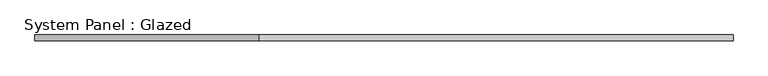
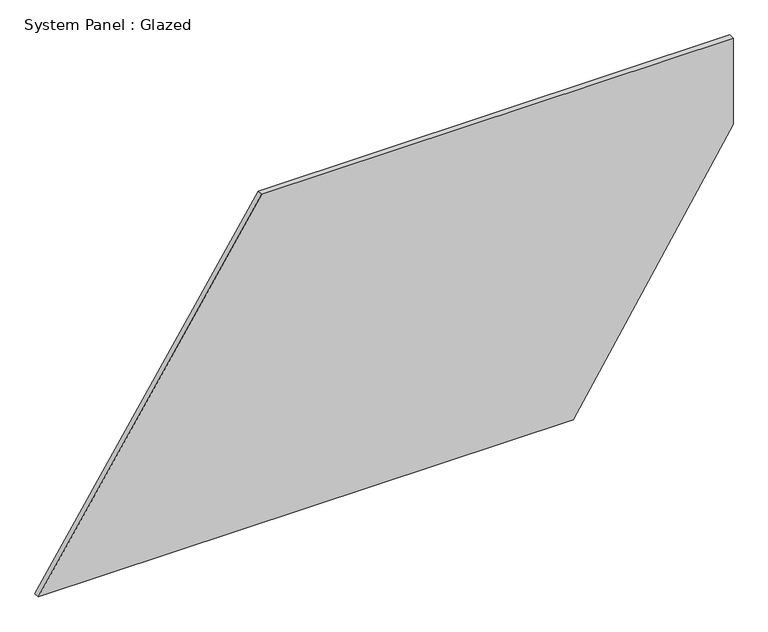
"""IFC4 building model written with IfcOpenShell, lengths in millimetres: plate geometry, System Panel : Glazed."""

import ifcopenshell
import ifcopenshell.guid

model = None  # the IFC model being written
_history = None  # IfcOwnerHistory: only IFC2X3 demands one
_inside = {}  # id of a spatial element -> (the spatial element, [elements in it])
_under = {}  # id of a project, library or spatial element -> (it, [spatial elements below it])
_declared = {}  # id of a project -> (the project, [libraries it declares])
_typed = {}  # id of a type object -> (the type object, [elements of that type])
_made_of = {}  # id of a material, layer set ... -> (it, [elements and type objects made of it])


def new_model(schema):
    """Start an empty IFC model of exactly this schema.

    Asked for "IFC4X3", IfcOpenShell would pick the latest addendum, in which some entities
    have other attributes; the version numbers below select the first issue.
    IFC2X3 requires an IfcOwnerHistory on every rooted entity: one is made here for all.
    """
    global model, _history
    if schema == "IFC4X3":
        model = ifcopenshell.file(schema_version=(4, 3, 0, 0))
    else:
        model = ifcopenshell.file(schema=schema)
    _inside.clear()
    _under.clear()
    _declared.clear()
    _typed.clear()
    _made_of.clear()
    _history = None
    if model.schema == "IFC2X3":
        org = make("IfcOrganization", Name="unknown")
        user = make(
            "IfcPersonAndOrganization",
            ThePerson=make("IfcPerson", FamilyName="unknown"),
            TheOrganization=org,
        )
        app = make(
            "IfcApplication",
            ApplicationDeveloper=org,
            Version="unknown",
            ApplicationFullName="unknown",
            ApplicationIdentifier="unknown",
        )
        _history = make(
            "IfcOwnerHistory",
            OwningUser=user,
            OwningApplication=app,
            ChangeAction="ADDED",
            CreationDate=0,
        )
    return model


def make(cls, **values):
    """One entity of the class cls with the attributes given. An attribute that is None is left unset."""
    return model.create_entity(
        cls, **{name: value for name, value in values.items() if value is not None}
    )


def rooted(cls, **values):
    """An entity with a GlobalId (a new one), such as an element, a storey or a relation."""
    return make(cls, GlobalId=ifcopenshell.guid.new(), OwnerHistory=_history, **values)


def si_unit(unit_type, name, prefix=None):
    """IfcSIUnit, for example si_unit("LENGTHUNIT", "METRE", prefix="MILLI")."""
    return make("IfcSIUnit", UnitType=unit_type, Prefix=prefix, Name=name)


def assignment(units):
    """IfcUnitAssignment: the units of a project."""
    return None if units is None else make("IfcUnitAssignment", Units=units)


def point(xyz):
    """IfcCartesianPoint."""
    return None if xyz is None else make("IfcCartesianPoint", Coordinates=xyz)


def direction(xyz):
    """IfcDirection."""
    return None if xyz is None else make("IfcDirection", DirectionRatios=xyz)


def frame(location, z_axis=None, x_axis=None):
    """IfcAxis2Placement3D, a coordinate frame: its origin and axes. An axis left out is left unset."""
    return make(
        "IfcAxis2Placement3D",
        Location=point(location),
        Axis=direction(z_axis),
        RefDirection=direction(x_axis),
    )


def origin():
    """The frame at (0, 0, 0) with its axes left unset."""
    return frame((0.0, 0.0, 0.0))


def place(relative_to, where):
    """IfcLocalPlacement: puts the frame where relative to a parent placement (None: the world)."""
    return make(
        "IfcLocalPlacement", PlacementRelTo=relative_to, RelativePlacement=where
    )


def context(
    kind, dimensions, precision=None, world=None, true_north=None, identifier=None
):
    """IfcGeometricRepresentationContext, for example the 3D "Model" context."""
    return make(
        "IfcGeometricRepresentationContext",
        ContextIdentifier=identifier,
        ContextType=kind,
        CoordinateSpaceDimension=dimensions,
        Precision=precision,
        WorldCoordinateSystem=world,
        TrueNorth=true_north,
    )


def project(units=None, contexts=None):
    """IfcProject with its units and contexts."""
    return rooted(
        "IfcProject",
        Name="project",
        RepresentationContexts=contexts,
        UnitsInContext=assignment(units),
    )


def spatial(cls, under=None, at=None, **own):
    """A site, building, storey or space (cls), placed at a placement, below another one or the project."""
    s = rooted(cls, ObjectPlacement=at, **own)
    if under is not None:
        _under.setdefault(under.id(), (under, []))[1].append(s)
    return s


def polyline(points):
    """IfcPolyline through the points."""
    return make("IfcPolyline", Points=[point(p) for p in points])


def outline(outer, holes=None, kind="AREA"):
    """IfcArbitraryClosedProfileDef: a profile drawn as a closed curve; with holes, ...WithVoids."""
    if holes is None:
        return make("IfcArbitraryClosedProfileDef", ProfileType=kind, OuterCurve=outer)
    return make(
        "IfcArbitraryProfileDefWithVoids",
        ProfileType=kind,
        OuterCurve=outer,
        InnerCurves=holes,
    )


def extrude(swept, where, along, depth):
    """IfcExtrudedAreaSolid: the profile swept, set in the frame where, extruded along a direction by depth."""
    return make(
        "IfcExtrudedAreaSolid",
        SweptArea=swept,
        Position=where,
        ExtrudedDirection=direction(along),
        Depth=depth,
    )


def shape(context_of_items, identifier, shape_type, items):
    """IfcShapeRepresentation: the items that make up one representation, for example the "Body"."""
    return make(
        "IfcShapeRepresentation",
        ContextOfItems=context_of_items,
        RepresentationIdentifier=identifier,
        RepresentationType=shape_type,
        Items=items,
    )


def source(mapping_origin, context_of_items, identifier, shape_type, items):
    """IfcRepresentationMap: a shape defined once, which mapped items show again and again."""
    return make(
        "IfcRepresentationMap",
        MappingOrigin=mapping_origin,
        MappedRepresentation=shape(context_of_items, identifier, shape_type, items),
    )


def transform(
    local_origin,
    x_axis=None,
    y_axis=None,
    z_axis=None,
    scale=None,
    scale2=None,
    scale3=None,
    uniform=True,
):
    """IfcCartesianTransformationOperator3D, or its non-uniform kind. x_axis, y_axis, z_axis: its Axis1, 2, 3."""
    if uniform:
        return make(
            "IfcCartesianTransformationOperator3D",
            Axis1=direction(x_axis),
            Axis2=direction(y_axis),
            LocalOrigin=point(local_origin),
            Scale=scale,
            Axis3=direction(z_axis),
        )
    return make(
        "IfcCartesianTransformationOperator3DnonUniform",
        Axis1=direction(x_axis),
        Axis2=direction(y_axis),
        LocalOrigin=point(local_origin),
        Scale=scale,
        Axis3=direction(z_axis),
        Scale2=scale2,
        Scale3=scale3,
    )


def mapped(mapping_source, mapping_target):
    """IfcMappedItem: shows the shape of a source again, moved by a transform."""
    return make(
        "IfcMappedItem", MappingSource=mapping_source, MappingTarget=mapping_target
    )


def made_of(thing, what):
    """Note that an element or type object is made of a material, layer set ...; save() writes the relation."""
    if what is not None:
        _made_of.setdefault(what.id(), (what, []))[1].append(thing)
    return thing


def element(
    cls,
    number,
    at=None,
    inside=None,
    cuts=None,
    type_object=None,
    material=None,
    context=None,
    identifier="Body",
    shape_type=None,
    held_by="IfcProductDefinitionShape",
    body=None,
    shapes=None,
    **own,
):
    """One element of the class cls, such as IfcWall. Its Tag is "e" and its number.

    at: its placement. inside: the storey or other place that contains it. cuts: it is an
    opening in that element (IfcRelVoidsElement). A single representation is given by context,
    identifier, shape_type and body (its items); several are given by shapes. held_by: the class
    of the entity that holds the representations. save() writes the other relations.
    """
    e = rooted(cls, Tag="e%d" % number, ObjectPlacement=at, **own)
    if body is not None:
        shapes = [shape(context, identifier, shape_type, body)]
    if shapes is not None:
        e.Representation = make(held_by, Representations=shapes)
    if inside is not None:
        _inside.setdefault(inside.id(), (inside, []))[1].append(e)
    if cuts is not None:
        rooted(
            "IfcRelVoidsElement", RelatingBuildingElement=cuts, RelatedOpeningElement=e
        )
    if type_object is not None:
        _typed.setdefault(type_object.id(), (type_object, []))[1].append(e)
    return made_of(e, material)


def aggregate(whole, parts):
    """IfcRelAggregates: a whole, such as a stair, and the parts it consists of."""
    return rooted("IfcRelAggregates", RelatingObject=whole, RelatedObjects=parts)


def save(model, path):
    """Write the relations noted so far, then the file.

    IfcRelAggregates (storeys below a building ...), IfcRelContainedInSpatialStructure (elements
    in a storey), IfcRelDefinesByType, IfcRelAssociatesMaterial and IfcRelDeclares: one each for
    every whole, place, type object, material and project.
    """
    for whole, parts in _under.values():
        aggregate(whole, parts)
    for where, things in _inside.values():
        rooted(
            "IfcRelContainedInSpatialStructure",
            RelatedElements=things,
            RelatingStructure=where,
        )
    for kind, things in _typed.values():
        rooted("IfcRelDefinesByType", RelatedObjects=things, RelatingType=kind)
    for what, things in _made_of.values():
        rooted("IfcRelAssociatesMaterial", RelatedObjects=things, RelatingMaterial=what)
    for by, libraries in _declared.values():
        rooted("IfcRelDeclares", RelatingContext=by, RelatedDefinitions=libraries)
    model.write(path)


def system_panel_glazed_eafb65c3(model_context):
    return source(origin(), model_context, "Body", "SweptSolid", [
        extrude(outline(polyline([(0.0, -1500.0000002), (0.0, 809.3899279), (1108.1997603, 1500.0000002), (1500.0, 1500.0000002), (1500.0, -535.7030249), (0.0, -1500.0000002)])), frame((0.0, 24.5, 0.0), z_axis=(0.0, 1.0, 0.0), x_axis=(0.0, 0.0, 1.0)), (0.0, 0.0, 1.0), 25.0),
    ])


if __name__ == "__main__":
    model = new_model("IFC4")
    model_context = context("Model", 3, world=origin())
    ifc_project = project(units=[si_unit("LENGTHUNIT", "METRE", prefix="MILLI")], contexts=[model_context])
    site = spatial("IfcSite", under=ifc_project)
    building = spatial("IfcBuilding", under=site)
    placement = place(None, origin())
    system_panel_glazed_shape = system_panel_glazed_eafb65c3(model_context)
    element("IfcPlate", 1, ObjectType="System Panel : Glazed", at=placement, inside=building, context=model_context, shape_type="MappedRepresentation", body=[
        mapped(system_panel_glazed_shape, transform((0.0, 0.0, 0.0), x_axis=(1.0, 0.0, 0.0), y_axis=(0.0, 1.0, 0.0), z_axis=(0.0, 0.0, 1.0))),
    ])
    save(model, "model.ifc")

# Revit data of these elements
# Type "System Panel : Glazed"
#   Construction Type Id = "GSP4R"
#   Analytic Construction = "1/8 in Pilkington single glazing"
#   Visual Light Transmittance = 0.9
#   Solar Heat Gain Coefficient = 0.86
#   Heat Transfer Coefficient (U) = 6.7069 W/(m²·K)
#   Define Thermal Properties by = 1
# Element 1 (IfcPlate, "System Panel : Glazed")
#   Materials on its faces: "Glass"
# Materials
#   "Glass": class "Glass", colour RGB 0 128 192, transparency 0.9, Description = "Soda Lime Glass", Cost = 0
